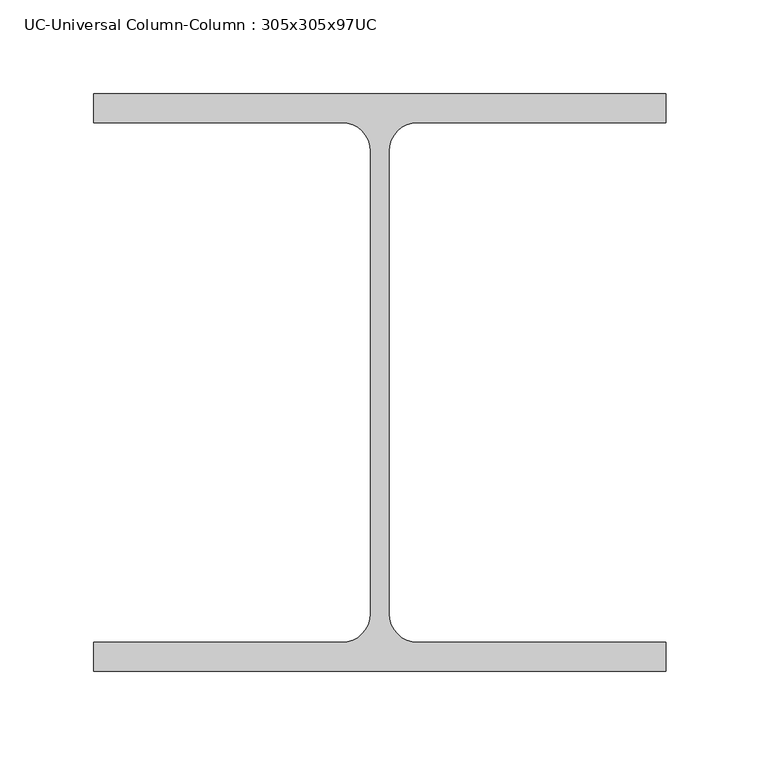
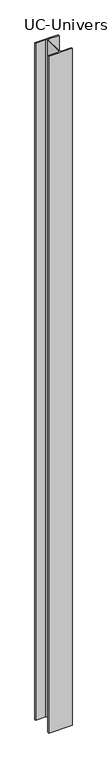
"""IFC4 building model written with IfcOpenShell, lengths in millimetres: column geometry, UC-Universal Column-Column : 305x305x97UC."""

import ifcopenshell
import ifcopenshell.guid

model = None  # the IFC model being written
_history = None  # IfcOwnerHistory: only IFC2X3 demands one
_inside = {}  # id of a spatial element -> (the spatial element, [elements in it])
_under = {}  # id of a project, library or spatial element -> (it, [spatial elements below it])
_declared = {}  # id of a project -> (the project, [libraries it declares])
_typed = {}  # id of a type object -> (the type object, [elements of that type])
_made_of = {}  # id of a material, layer set ... -> (it, [elements and type objects made of it])


def new_model(schema):
    """Start an empty IFC model of exactly this schema.

    Asked for "IFC4X3", IfcOpenShell would pick the latest addendum, in which some entities
    have other attributes; the version numbers below select the first issue.
    IFC2X3 requires an IfcOwnerHistory on every rooted entity: one is made here for all.
    """
    global model, _history
    if schema == "IFC4X3":
        model = ifcopenshell.file(schema_version=(4, 3, 0, 0))
    else:
        model = ifcopenshell.file(schema=schema)
    _inside.clear()
    _under.clear()
    _declared.clear()
    _typed.clear()
    _made_of.clear()
    _history = None
    if model.schema == "IFC2X3":
        org = make("IfcOrganization", Name="unknown")
        user = make(
            "IfcPersonAndOrganization",
            ThePerson=make("IfcPerson", FamilyName="unknown"),
            TheOrganization=org,
        )
        app = make(
            "IfcApplication",
            ApplicationDeveloper=org,
            Version="unknown",
            ApplicationFullName="unknown",
            ApplicationIdentifier="unknown",
        )
        _history = make(
            "IfcOwnerHistory",
            OwningUser=user,
            OwningApplication=app,
            ChangeAction="ADDED",
            CreationDate=0,
        )
    return model


def make(cls, **values):
    """One entity of the class cls with the attributes given. An attribute that is None is left unset."""
    return model.create_entity(
        cls, **{name: value for name, value in values.items() if value is not None}
    )


def rooted(cls, **values):
    """An entity with a GlobalId (a new one), such as an element, a storey or a relation."""
    return make(cls, GlobalId=ifcopenshell.guid.new(), OwnerHistory=_history, **values)


def si_unit(unit_type, name, prefix=None):
    """IfcSIUnit, for example si_unit("LENGTHUNIT", "METRE", prefix="MILLI")."""
    return make("IfcSIUnit", UnitType=unit_type, Prefix=prefix, Name=name)


def assignment(units):
    """IfcUnitAssignment: the units of a project."""
    return None if units is None else make("IfcUnitAssignment", Units=units)


def point(xyz):
    """IfcCartesianPoint."""
    return None if xyz is None else make("IfcCartesianPoint", Coordinates=xyz)


def direction(xyz):
    """IfcDirection."""
    return None if xyz is None else make("IfcDirection", DirectionRatios=xyz)


def frame(location, z_axis=None, x_axis=None):
    """IfcAxis2Placement3D, a coordinate frame: its origin and axes. An axis left out is left unset."""
    return make(
        "IfcAxis2Placement3D",
        Location=point(location),
        Axis=direction(z_axis),
        RefDirection=direction(x_axis),
    )


def frame_2d(location, x_axis=None):
    """IfcAxis2Placement2D, a coordinate frame in the plane: its origin and x axis."""
    return make(
        "IfcAxis2Placement2D", Location=point(location), RefDirection=direction(x_axis)
    )


def origin():
    """The frame at (0, 0, 0) with its axes left unset."""
    return frame((0.0, 0.0, 0.0))


def place(relative_to, where):
    """IfcLocalPlacement: puts the frame where relative to a parent placement (None: the world)."""
    return make(
        "IfcLocalPlacement", PlacementRelTo=relative_to, RelativePlacement=where
    )


def context(
    kind, dimensions, precision=None, world=None, true_north=None, identifier=None
):
    """IfcGeometricRepresentationContext, for example the 3D "Model" context."""
    return make(
        "IfcGeometricRepresentationContext",
        ContextIdentifier=identifier,
        ContextType=kind,
        CoordinateSpaceDimension=dimensions,
        Precision=precision,
        WorldCoordinateSystem=world,
        TrueNorth=true_north,
    )


def project(units=None, contexts=None):
    """IfcProject with its units and contexts."""
    return rooted(
        "IfcProject",
        Name="project",
        RepresentationContexts=contexts,
        UnitsInContext=assignment(units),
    )


def spatial(cls, under=None, at=None, **own):
    """A site, building, storey or space (cls), placed at a placement, below another one or the project."""
    s = rooted(cls, ObjectPlacement=at, **own)
    if under is not None:
        _under.setdefault(under.id(), (under, []))[1].append(s)
    return s


def polyline(points):
    """IfcPolyline through the points."""
    return make("IfcPolyline", Points=[point(p) for p in points])


def circle_curve(where, radius):
    """IfcCircle in the frame where."""
    return make("IfcCircle", Position=where, Radius=radius)


def trimmed(basis, trim1, trim2, sense, master):
    """IfcTrimmedCurve: the piece of a basis curve between two trims."""
    return make(
        "IfcTrimmedCurve",
        BasisCurve=basis,
        Trim1=trim1,
        Trim2=trim2,
        SenseAgreement=sense,
        MasterRepresentation=master,
    )


def segment(curve, same_sense, transition):
    """IfcCompositeCurveSegment."""
    return make(
        "IfcCompositeCurveSegment",
        Transition=transition,
        SameSense=same_sense,
        ParentCurve=curve,
    )


def composite_curve(segments, self_intersect=None):
    """IfcCompositeCurve: segments joined end to end."""
    return make("IfcCompositeCurve", Segments=segments, SelfIntersect=self_intersect)


def outline(outer, holes=None, kind="AREA"):
    """IfcArbitraryClosedProfileDef: a profile drawn as a closed curve; with holes, ...WithVoids."""
    if holes is None:
        return make("IfcArbitraryClosedProfileDef", ProfileType=kind, OuterCurve=outer)
    return make(
        "IfcArbitraryProfileDefWithVoids",
        ProfileType=kind,
        OuterCurve=outer,
        InnerCurves=holes,
    )


def extrude(swept, where, along, depth):
    """IfcExtrudedAreaSolid: the profile swept, set in the frame where, extruded along a direction by depth."""
    return make(
        "IfcExtrudedAreaSolid",
        SweptArea=swept,
        Position=where,
        ExtrudedDirection=direction(along),
        Depth=depth,
    )


def shape(context_of_items, identifier, shape_type, items):
    """IfcShapeRepresentation: the items that make up one representation, for example the "Body"."""
    return make(
        "IfcShapeRepresentation",
        ContextOfItems=context_of_items,
        RepresentationIdentifier=identifier,
        RepresentationType=shape_type,
        Items=items,
    )


def source(mapping_origin, context_of_items, identifier, shape_type, items):
    """IfcRepresentationMap: a shape defined once, which mapped items show again and again."""
    return make(
        "IfcRepresentationMap",
        MappingOrigin=mapping_origin,
        MappedRepresentation=shape(context_of_items, identifier, shape_type, items),
    )


def transform(
    local_origin,
    x_axis=None,
    y_axis=None,
    z_axis=None,
    scale=None,
    scale2=None,
    scale3=None,
    uniform=True,
):
    """IfcCartesianTransformationOperator3D, or its non-uniform kind. x_axis, y_axis, z_axis: its Axis1, 2, 3."""
    if uniform:
        return make(
            "IfcCartesianTransformationOperator3D",
            Axis1=direction(x_axis),
            Axis2=direction(y_axis),
            LocalOrigin=point(local_origin),
            Scale=scale,
            Axis3=direction(z_axis),
        )
    return make(
        "IfcCartesianTransformationOperator3DnonUniform",
        Axis1=direction(x_axis),
        Axis2=direction(y_axis),
        LocalOrigin=point(local_origin),
        Scale=scale,
        Axis3=direction(z_axis),
        Scale2=scale2,
        Scale3=scale3,
    )


def mapped(mapping_source, mapping_target):
    """IfcMappedItem: shows the shape of a source again, moved by a transform."""
    return make(
        "IfcMappedItem", MappingSource=mapping_source, MappingTarget=mapping_target
    )


def made_of(thing, what):
    """Note that an element or type object is made of a material, layer set ...; save() writes the relation."""
    if what is not None:
        _made_of.setdefault(what.id(), (what, []))[1].append(thing)
    return thing


def element(
    cls,
    number,
    at=None,
    inside=None,
    cuts=None,
    type_object=None,
    material=None,
    context=None,
    identifier="Body",
    shape_type=None,
    held_by="IfcProductDefinitionShape",
    body=None,
    shapes=None,
    **own,
):
    """One element of the class cls, such as IfcWall. Its Tag is "e" and its number.

    at: its placement. inside: the storey or other place that contains it. cuts: it is an
    opening in that element (IfcRelVoidsElement). A single representation is given by context,
    identifier, shape_type and body (its items); several are given by shapes. held_by: the class
    of the entity that holds the representations. save() writes the other relations.
    """
    e = rooted(cls, Tag="e%d" % number, ObjectPlacement=at, **own)
    if body is not None:
        shapes = [shape(context, identifier, shape_type, body)]
    if shapes is not None:
        e.Representation = make(held_by, Representations=shapes)
    if inside is not None:
        _inside.setdefault(inside.id(), (inside, []))[1].append(e)
    if cuts is not None:
        rooted(
            "IfcRelVoidsElement", RelatingBuildingElement=cuts, RelatedOpeningElement=e
        )
    if type_object is not None:
        _typed.setdefault(type_object.id(), (type_object, []))[1].append(e)
    return made_of(e, material)


def aggregate(whole, parts):
    """IfcRelAggregates: a whole, such as a stair, and the parts it consists of."""
    return rooted("IfcRelAggregates", RelatingObject=whole, RelatedObjects=parts)


def save(model, path):
    """Write the relations noted so far, then the file.

    IfcRelAggregates (storeys below a building ...), IfcRelContainedInSpatialStructure (elements
    in a storey), IfcRelDefinesByType, IfcRelAssociatesMaterial and IfcRelDeclares: one each for
    every whole, place, type object, material and project.
    """
    for whole, parts in _under.values():
        aggregate(whole, parts)
    for where, things in _inside.values():
        rooted(
            "IfcRelContainedInSpatialStructure",
            RelatedElements=things,
            RelatingStructure=where,
        )
    for kind, things in _typed.values():
        rooted("IfcRelDefinesByType", RelatedObjects=things, RelatingType=kind)
    for what, things in _made_of.values():
        rooted("IfcRelAssociatesMaterial", RelatedObjects=things, RelatingMaterial=what)
    for by, libraries in _declared.values():
        rooted("IfcRelDeclares", RelatingContext=by, RelatedDefinitions=libraries)
    model.write(path)


def uc_universal_column_column_305x305x97uc_8da79b43(model_context):
    return source(origin(), model_context, "Body", "SweptSolid", [
        extrude(outline(composite_curve([segment(polyline([(152.65, -153.95), (-152.65, -153.95), (-152.65, -138.55), (-20.15, -138.55)]), True, "CONTINUOUS"), segment(trimmed(circle_curve(frame_2d((-20.15, -123.35)), 15.2), [point((-20.15, -138.55))], [point((-4.95, -123.35))], True, "CARTESIAN"), True, "CONTINUOUS"), segment(polyline([(-4.95, -123.35), (-4.95, 123.35)]), True, "CONTINUOUS"), segment(trimmed(circle_curve(frame_2d((-20.15, 123.35)), 15.2), [point((-4.95, 123.35))], [point((-20.15, 138.55))], True, "CARTESIAN"), True, "CONTINUOUS"), segment(polyline([(-20.15, 138.55), (-152.65, 138.55), (-152.65, 153.95), (152.65, 153.95), (152.65, 138.55), (20.15, 138.55)]), True, "CONTINUOUS"), segment(trimmed(circle_curve(frame_2d((20.15, 123.35)), 15.2), [point((20.15, 138.55))], [point((4.95, 123.35))], True, "CARTESIAN"), True, "CONTINUOUS"), segment(polyline([(4.95, 123.35), (4.95, -123.35)]), True, "CONTINUOUS"), segment(trimmed(circle_curve(frame_2d((20.15, -123.35)), 15.2), [point((4.95, -123.35))], [point((20.15, -138.55))], True, "CARTESIAN"), True, "CONTINUOUS"), segment(polyline([(20.15, -138.55), (152.65, -138.55), (152.65, -153.95)]), True, "CONTINUOUS")], self_intersect=False)), frame((0.0, 0.0, -1500.0), z_axis=(0.0, 0.0, 1.0), x_axis=(1.0, 0.0, 0.0)), (0.0, 0.0, 1.0), 9300.0),
    ])


if __name__ == "__main__":
    model = new_model("IFC4")
    model_context = context("Model", 3, world=origin())
    ifc_project = project(units=[si_unit("LENGTHUNIT", "METRE", prefix="MILLI")], contexts=[model_context])
    site = spatial("IfcSite", under=ifc_project)
    building = spatial("IfcBuilding", under=site)
    placement = place(None, origin())
    uc_universal_column_column_305x305x97uc_shape = uc_universal_column_column_305x305x97uc_8da79b43(model_context)
    element("IfcColumn", 1, ObjectType="UC-Universal Column-Column : 305x305x97UC", at=placement, inside=building, context=model_context, shape_type="MappedRepresentation", body=[
        mapped(uc_universal_column_column_305x305x97uc_shape, transform((0.0, 0.0, 0.0), x_axis=(1.0, 0.0, 0.0), y_axis=(0.0, 1.0, 0.0), z_axis=(0.0, 0.0, 1.0))),
    ])
    save(model, "model.ifc")

# Revit data of these elements
# Type "UC-Universal Column-Column : 305x305x97UC"
#   Keynote = "G10"
#   Nominal h = ""
#   W = 0
#   Ix = 0
#   M = 96.9
#   Zx = 0
#   b = 305.3 mm
#   h = 307.9 mm
#   r = 15.2 mm
#   s = 9.9 mm
#   t = 15.4 mm
#   A = 123 m²
#   Structural Material [instance default] = Steel, 45-345
#   Assembly Code = ""
# Element 1 (IfcColumn, "UC-Universal Column-Column : 305x305x97UC")
#   Materials on its faces: "Steel, 45-345"
# Materials
#   "Steel, 45-345": class "Metal", colour RGB 247 247 247, transparency 0, Description = "Steel 345 MPa", Cost = 0
